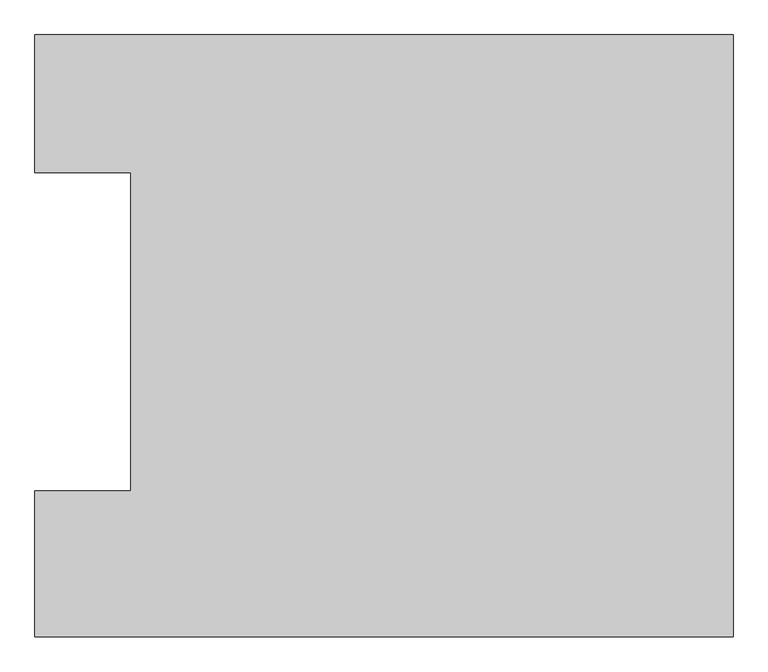
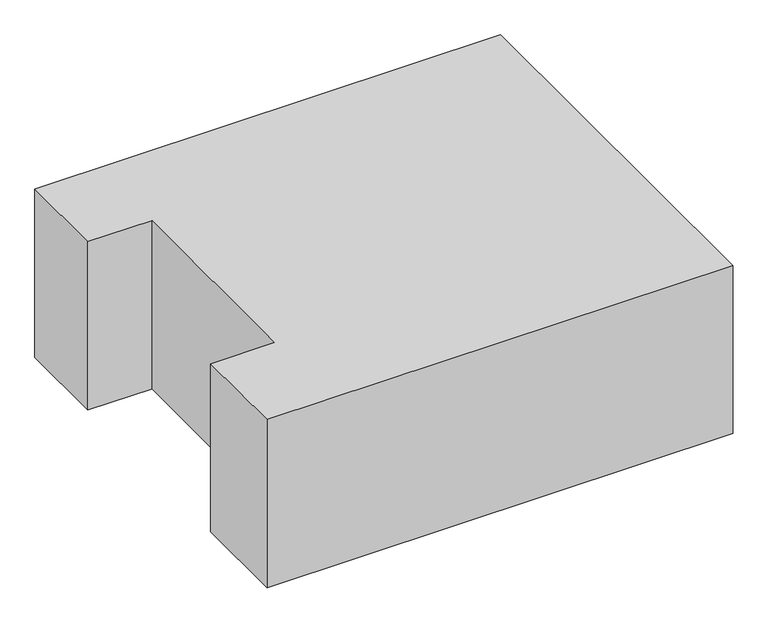
"""IFC4 building model written with IfcOpenShell, lengths in millimetres: proxy geometry, 0_3d_modell."""

from ifc_helpers import new_model, si_unit, origin, origin_with_axes, place, context, project, spatial, polyline, outline, extrude, source, transform, mapped, element, save


def generic_models_1e1fada3(model_context):
    return source(origin(), model_context, "Body", "SweptSolid", [
        extrude(outline(polyline([(0.0, 0.0), (0.0, 1367.8), (900.0, 1367.8), (900.0, 4357.8), (0.0, 4357.8), (0.0, 5650.0), (6550.0, 5650.0), (6550.0, 0.0), (0.0, 0.0)])), origin_with_axes(), (0.0, 0.0, 1.0), 2500.0),
    ])


if __name__ == "__main__":
    model = new_model("IFC4")
    model_context = context("Model", 3, world=origin())
    ifc_project = project(units=[si_unit("LENGTHUNIT", "METRE", prefix="MILLI")], contexts=[model_context])
    site = spatial("IfcSite", under=ifc_project)
    building = spatial("IfcBuilding", under=site)
    placement = place(None, origin())
    generic_models_shape = generic_models_1e1fada3(model_context)
    element("IfcBuildingElementProxy", 1, Name="0_3d_modell", ObjectType="0_3d_modell", at=placement, inside=building, context=model_context, shape_type="MappedRepresentation", body=[
        mapped(generic_models_shape, transform((0.0, 0.0, 0.0), x_axis=(1.0, 0.0, 0.0), y_axis=(0.0, 1.0, 0.0), z_axis=(0.0, 0.0, 1.0))),
    ])
    save(model, "model.ifc")

# Revit data of these elements
# Element 1 (IfcBuildingElementProxy, "0_3d_modell")
#   Materials on its faces: "*1"
# Materials
#   "*1": class "Unassigned", colour RGB 175 175 175, transparency 0
